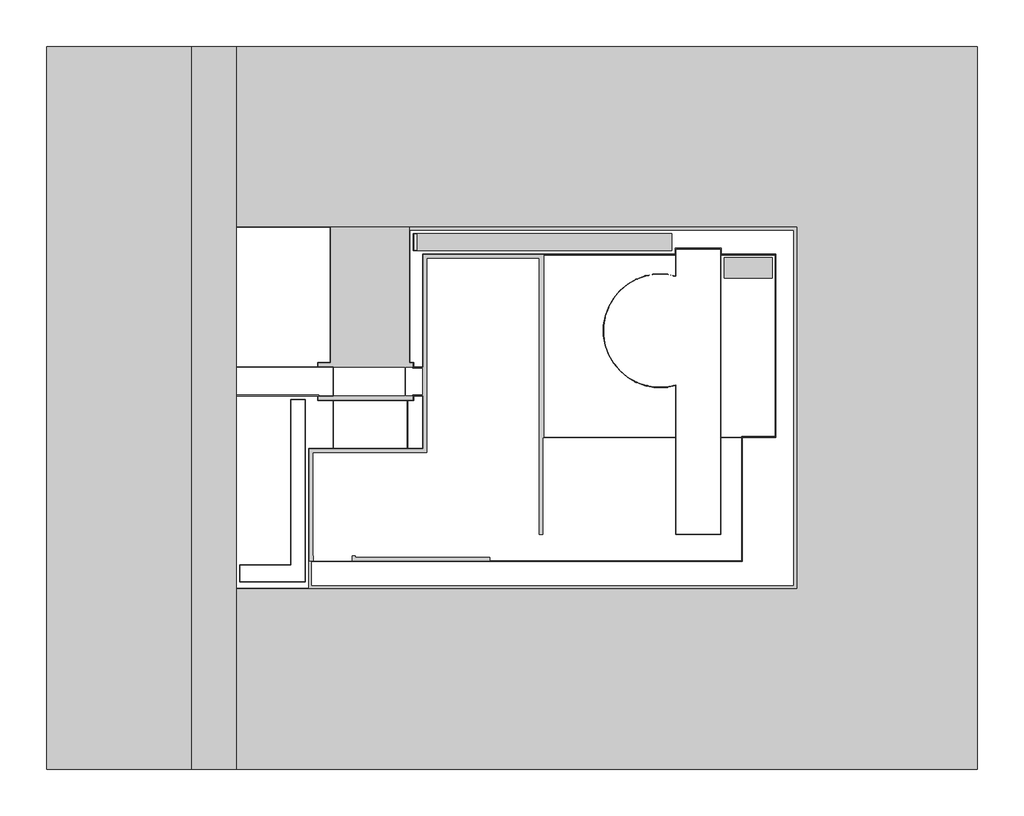
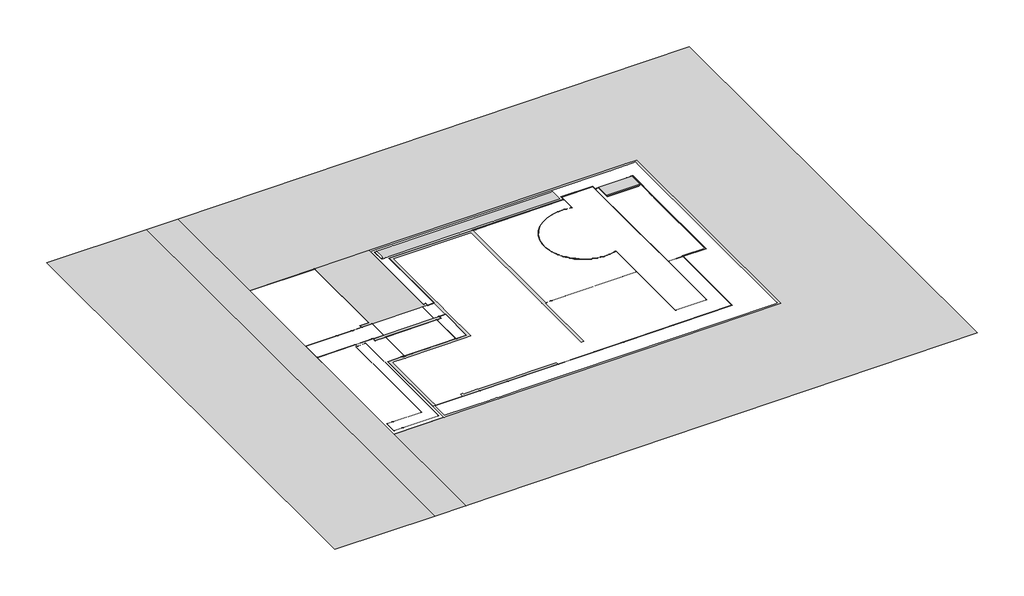
# One storey: 11 proxies.
"""IFC4 building model written with IfcOpenShell, lengths in millimetres."""

import ifcopenshell
import ifcopenshell.guid

model = None  # the IFC model being written
_history = None  # IfcOwnerHistory: only IFC2X3 demands one
_inside = {}  # id of a spatial element -> (the spatial element, [elements in it])
_under = {}  # id of a project, library or spatial element -> (it, [spatial elements below it])
_declared = {}  # id of a project -> (the project, [libraries it declares])
_typed = {}  # id of a type object -> (the type object, [elements of that type])
_made_of = {}  # id of a material, layer set ... -> (it, [elements and type objects made of it])


def new_model(schema):
    """Start an empty IFC model of exactly this schema.

    Asked for "IFC4X3", IfcOpenShell would pick the latest addendum, in which some entities
    have other attributes; the version numbers below select the first issue.
    IFC2X3 requires an IfcOwnerHistory on every rooted entity: one is made here for all.
    """
    global model, _history
    if schema == "IFC4X3":
        model = ifcopenshell.file(schema_version=(4, 3, 0, 0))
    else:
        model = ifcopenshell.file(schema=schema)
    _inside.clear()
    _under.clear()
    _declared.clear()
    _typed.clear()
    _made_of.clear()
    _history = None
    if model.schema == "IFC2X3":
        org = make("IfcOrganization", Name="unknown")
        user = make(
            "IfcPersonAndOrganization",
            ThePerson=make("IfcPerson", FamilyName="unknown"),
            TheOrganization=org,
        )
        app = make(
            "IfcApplication",
            ApplicationDeveloper=org,
            Version="unknown",
            ApplicationFullName="unknown",
            ApplicationIdentifier="unknown",
        )
        _history = make(
            "IfcOwnerHistory",
            OwningUser=user,
            OwningApplication=app,
            ChangeAction="ADDED",
            CreationDate=0,
        )
    return model


def make(cls, **values):
    """One entity of the class cls with the attributes given. An attribute that is None is left unset."""
    return model.create_entity(
        cls, **{name: value for name, value in values.items() if value is not None}
    )


def rooted(cls, **values):
    """An entity with a GlobalId (a new one), such as an element, a storey or a relation."""
    return make(cls, GlobalId=ifcopenshell.guid.new(), OwnerHistory=_history, **values)


def si_unit(unit_type, name, prefix=None):
    """IfcSIUnit, for example si_unit("LENGTHUNIT", "METRE", prefix="MILLI")."""
    return make("IfcSIUnit", UnitType=unit_type, Prefix=prefix, Name=name)


def assignment(units):
    """IfcUnitAssignment: the units of a project."""
    return None if units is None else make("IfcUnitAssignment", Units=units)


def point(xyz):
    """IfcCartesianPoint."""
    return None if xyz is None else make("IfcCartesianPoint", Coordinates=xyz)


def direction(xyz):
    """IfcDirection."""
    return None if xyz is None else make("IfcDirection", DirectionRatios=xyz)


def frame(location, z_axis=None, x_axis=None):
    """IfcAxis2Placement3D, a coordinate frame: its origin and axes. An axis left out is left unset."""
    return make(
        "IfcAxis2Placement3D",
        Location=point(location),
        Axis=direction(z_axis),
        RefDirection=direction(x_axis),
    )


def origin():
    """The frame at (0, 0, 0) with its axes left unset."""
    return frame((0.0, 0.0, 0.0))


def place(relative_to, where):
    """IfcLocalPlacement: puts the frame where relative to a parent placement (None: the world)."""
    return make(
        "IfcLocalPlacement", PlacementRelTo=relative_to, RelativePlacement=where
    )


def context(
    kind, dimensions, precision=None, world=None, true_north=None, identifier=None
):
    """IfcGeometricRepresentationContext, for example the 3D "Model" context."""
    return make(
        "IfcGeometricRepresentationContext",
        ContextIdentifier=identifier,
        ContextType=kind,
        CoordinateSpaceDimension=dimensions,
        Precision=precision,
        WorldCoordinateSystem=world,
        TrueNorth=true_north,
    )


def project(units=None, contexts=None):
    """IfcProject with its units and contexts."""
    return rooted(
        "IfcProject",
        Name="project",
        RepresentationContexts=contexts,
        UnitsInContext=assignment(units),
    )


def spatial(cls, under=None, at=None, **own):
    """A site, building, storey or space (cls), placed at a placement, below another one or the project."""
    s = rooted(cls, ObjectPlacement=at, **own)
    if under is not None:
        _under.setdefault(under.id(), (under, []))[1].append(s)
    return s


def polyline(points):
    """IfcPolyline through the points."""
    return make("IfcPolyline", Points=[point(p) for p in points])


def point_list(points):
    """IfcCartesianPointList2D or 3D."""
    cls = (
        "IfcCartesianPointList2D" if len(points[0]) == 2 else "IfcCartesianPointList3D"
    )
    return make(cls, CoordList=points)


def outline(outer, holes=None, kind="AREA"):
    """IfcArbitraryClosedProfileDef: a profile drawn as a closed curve; with holes, ...WithVoids."""
    if holes is None:
        return make("IfcArbitraryClosedProfileDef", ProfileType=kind, OuterCurve=outer)
    return make(
        "IfcArbitraryProfileDefWithVoids",
        ProfileType=kind,
        OuterCurve=outer,
        InnerCurves=holes,
    )


def extrude(swept, where, along, depth):
    """IfcExtrudedAreaSolid: the profile swept, set in the frame where, extruded along a direction by depth."""
    return make(
        "IfcExtrudedAreaSolid",
        SweptArea=swept,
        Position=where,
        ExtrudedDirection=direction(along),
        Depth=depth,
    )


def triangles(points, corners, closed=None, point_numbers=None):
    """IfcTriangulatedFaceSet: each triangle names its three corners, points numbered from 1."""
    return make(
        "IfcTriangulatedFaceSet",
        Coordinates=point_list(points),
        Closed=closed,
        CoordIndex=corners,
        PnIndex=point_numbers,
    )


def shape(context_of_items, identifier, shape_type, items):
    """IfcShapeRepresentation: the items that make up one representation, for example the "Body"."""
    return make(
        "IfcShapeRepresentation",
        ContextOfItems=context_of_items,
        RepresentationIdentifier=identifier,
        RepresentationType=shape_type,
        Items=items,
    )


def source(mapping_origin, context_of_items, identifier, shape_type, items):
    """IfcRepresentationMap: a shape defined once, which mapped items show again and again."""
    return make(
        "IfcRepresentationMap",
        MappingOrigin=mapping_origin,
        MappedRepresentation=shape(context_of_items, identifier, shape_type, items),
    )


def transform(
    local_origin,
    x_axis=None,
    y_axis=None,
    z_axis=None,
    scale=None,
    scale2=None,
    scale3=None,
    uniform=True,
):
    """IfcCartesianTransformationOperator3D, or its non-uniform kind. x_axis, y_axis, z_axis: its Axis1, 2, 3."""
    if uniform:
        return make(
            "IfcCartesianTransformationOperator3D",
            Axis1=direction(x_axis),
            Axis2=direction(y_axis),
            LocalOrigin=point(local_origin),
            Scale=scale,
            Axis3=direction(z_axis),
        )
    return make(
        "IfcCartesianTransformationOperator3DnonUniform",
        Axis1=direction(x_axis),
        Axis2=direction(y_axis),
        LocalOrigin=point(local_origin),
        Scale=scale,
        Axis3=direction(z_axis),
        Scale2=scale2,
        Scale3=scale3,
    )


def mapped(mapping_source, mapping_target):
    """IfcMappedItem: shows the shape of a source again, moved by a transform."""
    return make(
        "IfcMappedItem", MappingSource=mapping_source, MappingTarget=mapping_target
    )


def made_of(thing, what):
    """Note that an element or type object is made of a material, layer set ...; save() writes the relation."""
    if what is not None:
        _made_of.setdefault(what.id(), (what, []))[1].append(thing)
    return thing


def element(
    cls,
    number,
    at=None,
    inside=None,
    cuts=None,
    type_object=None,
    material=None,
    context=None,
    identifier="Body",
    shape_type=None,
    held_by="IfcProductDefinitionShape",
    body=None,
    shapes=None,
    **own,
):
    """One element of the class cls, such as IfcWall. Its Tag is "e" and its number.

    at: its placement. inside: the storey or other place that contains it. cuts: it is an
    opening in that element (IfcRelVoidsElement). A single representation is given by context,
    identifier, shape_type and body (its items); several are given by shapes. held_by: the class
    of the entity that holds the representations. save() writes the other relations.
    """
    e = rooted(cls, Tag="e%d" % number, ObjectPlacement=at, **own)
    if body is not None:
        shapes = [shape(context, identifier, shape_type, body)]
    if shapes is not None:
        e.Representation = make(held_by, Representations=shapes)
    if inside is not None:
        _inside.setdefault(inside.id(), (inside, []))[1].append(e)
    if cuts is not None:
        rooted(
            "IfcRelVoidsElement", RelatingBuildingElement=cuts, RelatedOpeningElement=e
        )
    if type_object is not None:
        _typed.setdefault(type_object.id(), (type_object, []))[1].append(e)
    return made_of(e, material)


def aggregate(whole, parts):
    """IfcRelAggregates: a whole, such as a stair, and the parts it consists of."""
    return rooted("IfcRelAggregates", RelatingObject=whole, RelatedObjects=parts)


def save(model, path):
    """Write the relations noted so far, then the file.

    IfcRelAggregates (storeys below a building ...), IfcRelContainedInSpatialStructure (elements
    in a storey), IfcRelDefinesByType, IfcRelAssociatesMaterial and IfcRelDeclares: one each for
    every whole, place, type object, material and project.
    """
    for whole, parts in _under.values():
        aggregate(whole, parts)
    for where, things in _inside.values():
        rooted(
            "IfcRelContainedInSpatialStructure",
            RelatedElements=things,
            RelatingStructure=where,
        )
    for kind, things in _typed.values():
        rooted("IfcRelDefinesByType", RelatedObjects=things, RelatingType=kind)
    for what, things in _made_of.values():
        rooted("IfcRelAssociatesMaterial", RelatedObjects=things, RelatingMaterial=what)
    for by, libraries in _declared.values():
        rooted("IfcRelDeclares", RelatingContext=by, RelatedDefinitions=libraries)
    model.write(path)


def specialty_equipment_67e2e29c(model_context):
    return source(origin(), model_context, "Body", "SweptSolid", [
        extrude(outline(polyline([(12687.718693, 5627.4300153), (12687.718693, 4481.4300153), (10041.718693, 4481.4300153), (10041.718693, 5627.4300153), (12687.718693, 5627.4300153)])), frame((0.0, 0.0, 280.0), z_axis=(0.0, 0.0, 1.0), x_axis=(1.0, 0.0, 0.0)), (0.0, 0.0, 1.0), 88.4706632),
        extrude(outline(polyline([(12614.718693, 5554.4300153), (12614.718693, 4554.4300153), (10114.718693, 4554.4300153), (10114.718693, 5554.4300153), (12614.718693, 5554.4300153)])), frame((0.0, 0.0, 200.0), z_axis=(0.0, 0.0, 1.0), x_axis=(1.0, 0.0, 0.0)), (0.0, 0.0, 1.0), 80.0),
    ])


model = new_model("IFC4")

# Units and contexts
model_context = context("Model", 3, world=origin())
ifc_project = project(units=[si_unit("LENGTHUNIT", "METRE", prefix="MILLI")], contexts=[model_context])

# Site, building, storey
site = spatial("IfcSite", under=ifc_project)
building = spatial("IfcBuilding", under=site)
storey = spatial("IfcBuildingStorey", under=building, Name="NÍVEL DA RUA", Elevation=0.0)

# Proxies
placement = place(None, origin())
element("IfcBuildingElementProxy", 1, Name="Building Element Proxy", at=placement, inside=storey, context=model_context, shape_type="Tessellation", body=[
    triangles([(24039.718689, -22695.5705017, 300.0000023), (24039.718689, 17304.4298035, 300.0000023), (-16960.2810425, 17304.4298035, 17.2413792), (-16960.2810425, 16538.146344, 17.2413792), (-16960.2810425, 7304.4297272, 17.2413792), (13164.7185333, 7304.4297272, 225.0000017), (14039.7186127, 7304.4297272, 231.0344808), (14039.7186127, -12695.5704254, 231.0344808), (-8585.2811966, -12695.5704254, 75.0000006), (-16960.2810425, -12695.5704254, 17.2413792), (-16960.2810425, -20396.7201233, 17.2413792), (-16960.2810425, -22695.5705017, 17.2413792)], [[11, 9, 10], [9, 11, 12], [6, 3, 4], [6, 4, 5], [12, 8, 9], [8, 12, 1], [8, 1, 7], [6, 7, 2], [2, 7, 1], [2, 3, 6]], closed=False),
])
element("IfcBuildingElementProxy", 2, Name="Building Element Proxy", at=placement, inside=storey, context=model_context, shape_type="Tessellation", body=[
    triangles([(-27460.2819946, 17304.4298035, 0.0), (-27460.2819946, -22695.5705017, 0.0), (-19460.2807709, -22695.5705017, 0.0), (-19460.2807709, -15076.5227692, 13.1362894), (-19460.2807709, 161.5728776, 13.1362894), (-19460.2807709, 9685.3826523, 13.1362894), (-19460.2807709, 17304.4298035, 0.0)], [[1, 2, 5], [5, 2, 4], [1, 5, 6], [3, 4, 2], [6, 7, 1]], closed=False),
])
element("IfcBuildingElementProxy", 3, Name="Building Element Proxy", at=placement, inside=storey, context=model_context, shape_type="Tessellation", body=[
    triangles([(-19460.2807709, -22695.5705017, 0.0), (-16960.2810425, -22695.5705017, 17.2413792), (-16960.2810425, -20396.7201233, 17.2413792), (-16960.2810425, -12695.5704254, 17.2413792), (-16960.2810425, 7304.4297272, 17.2413792), (-16960.2810425, 16538.146344, 17.2413792), (-16960.2810425, 17304.4298035, 17.2413792), (-19460.2807709, 17304.4298035, 0.0), (-19460.2807709, 9685.3826523, 13.1362894), (-19460.2807709, 161.5728776, 13.1362894), (-19460.2807709, -15076.5227692, 13.1362894)], [[10, 11, 4], [6, 8, 9], [5, 9, 10], [11, 1, 3], [11, 3, 4], [3, 1, 2], [6, 7, 8], [6, 9, 5], [4, 5, 10]], closed=False),
])
element("IfcBuildingElementProxy", 4, Name="Building Element Proxy", at=placement, inside=storey, context=model_context, shape_type="Tessellation", body=[
    triangles([(14039.7186127, 7304.4297272, 231.0344808), (13164.7185333, 7304.4297272, 225.0000017), (-7360.2815506, 7304.4297272, 83.4482767), (-7360.2815506, 7054.4298706, 83.4482767), (-7360.2815506, -195.5699849, 83.4482767), (-7160.2815491, -195.5699849, 84.8275893), (-7160.2815491, -445.5699686, 84.8275893), (-6660.2812546, -445.5699686, 88.2758617), (-6660.2812546, 5804.4300064, 88.2758617), (39.7186921, 5804.4300064, 134.4827615), (7339.7188522, 5804.4300064, 184.827581), (7339.7188522, 6104.4302994, 184.827581), (9839.719162, 6104.4302994, 202.0689704), (9839.719162, 5804.4300064, 202.0689704), (12414.7189636, 5804.4300064, 219.8275885), (12736.6074554, 5804.4300064, 222.0475111), (12889.7190399, 5804.4300064, 223.1034423), (12889.7190399, 5796.7827988, 223.1034423), (12889.7190399, 2838.5967934, 223.1034423), (12889.7190399, -4345.5699257, 223.1034423), (11039.7191711, -4345.5699257, 210.3448279), (11039.7191711, -11195.5701233, 210.3448279), (-6954.0313477, -11195.5701233, 86.2500043), (-9213.4062286, -11195.5701233, 70.668102), (-12960.281012, -11195.5701233, 44.8275872), (-12960.281012, -4945.5702209, 44.8275872), (-11830.5941528, -4945.5702209, 52.618536), (-11610.2808563, -4945.5702209, 54.1379291), (-11610.2808563, -4820.5615723, 54.1379291), (-11610.2808563, -2295.5700554, 54.1379291), (-12460.2812988, -2295.5700554, 48.2758642), (-12460.2812988, -2045.5700535, 48.2758642), (-13907.2197235, -2045.5700535, 38.296972), (-16960.2810425, -2045.5700535, 17.2413792), (-16960.2810425, -12695.5704254, 17.2413792), (-8585.2811966, -12695.5704254, 75.0000006), (14039.7186127, -12695.5704254, 231.0344808), (-12461.2812378, -2046.5183968, 48.2689651), (-12461.2812378, -2051.3699902, 48.2689651), (-12461.2812378, -2296.5699944, 48.2689651), (-12460.4696594, -2296.5699944, 48.2745606), (-11611.2807953, -2296.5699944, 54.1310346), (-11611.2807953, -4821.1289795, 54.1310346), (-11611.2807953, -4944.5697006, 54.1310346), (-11828.8314697, -4944.5697006, 52.6306901), (-11830.8313477, -4944.5697006, 52.6168964), (-12960.0926514, -4944.5697006, 44.8288862), (-12961.2809509, -4944.5697006, 44.8206881), (-12961.2809509, -4947.507312, 44.8206881), (-12961.2809509, -11195.944519, 44.8206881), (-12961.2809509, -12694.5704865, 44.8206881), (-16957.6149261, -12694.5704865, 17.2597704), (-16959.2811035, -12694.5704865, 17.2482761), (-16959.2811035, -12693.6321716, 17.2482761), (-16959.2811035, -2046.5183968, 17.2482761), (-13906.9104401, -2046.5183968, 38.2991112), (13889.7184662, 7154.430162, 230.0000054), (13889.7184662, 6721.9298172, 230.0000054), (13889.7184662, -12278.0703278, 230.0000054), (13889.7184662, -12545.5702789, 230.0000054), (13739.7183197, -12545.5702789, 228.9655118), (-6622.781218, -12545.5702789, 88.5344851), (-8422.1562698, -12545.5702789, 76.125), (-8648.0936417, -12545.5702789, 74.5668103), (-9022.7812363, -12545.5702789, 71.9827565), (-12809.2809265, -12545.5702789, 45.8689662), (-12809.2809265, -11247.3413818, 45.8689662), (-12809.2809265, -11196.5700623, 45.8689662), (-9212.9876495, -11196.5700623, 70.6709906), (-6955.119072, -11196.5700623, 86.2425011), (9.7186928, -11196.5700623, 134.275861), (2289.7186684, -11196.5700623, 150.0000011), (6259.7184952, -11196.5700623, 177.3793074), (11026.6350861, -11196.5700623, 210.25459), (11040.7191101, -11196.5700623, 210.3517316), (11040.7191101, -4348.353186, 210.3517316), (11040.7191101, -4346.5698647, 210.3517316), (12890.7189789, -4346.5698647, 223.110346), (12890.7189789, 2842.4799866, 223.110346), (12890.7189789, 5802.2650223, 223.110346), (12890.7189789, 5805.4299454, 223.110346), (12736.8923218, 5805.4299454, 222.0494732), (12415.2189331, 5805.4299454, 219.8310403), (9870.7184326, 5805.4299454, 202.2827655), (9870.7184326, 6135.4301514, 202.2827655), (7308.7184189, 6135.4301514, 184.6137859), (7308.7184189, 5805.4299454, 184.6137859), (48.468694, 5805.4299454, 134.5431049), (34.7853586, 5805.4299454, 134.4487338), (-6661.2811935, 5805.4299454, 88.2689672), (-6661.2811935, 5795.8584366, 88.2689672), (-6661.2811935, 5792.4301575, 88.2689672), (-6661.2811935, -444.5699933, 88.2689672), (-6662.2811325, -444.5699933, 88.2620726), (-7159.2810287, -444.5699933, 84.8344839), (-7159.2810287, -196.0699907, 84.8344839), (-7159.2810287, -194.5699914, 84.8344839), (-7160.1978333, -194.5699914, 84.8281616), (-7359.2810303, -194.5699914, 83.4551713), (-7359.2810303, -186.9985604, 83.4551713), (-7359.2810303, 7154.430162, 83.4551713), (-7290.2811722, 7154.430162, 83.9310325), (-6620.2813705, 7154.430162, 88.5517261), (11852.2184143, 7154.430162, 215.9482831), (13089.7184601, 7154.430162, 224.4827549), (13121.907193, 7154.430162, 224.7047436), (13137.3585754, 7154.430162, 224.8113141), (-12460.2812988, -445.5699686, 48.2758642), (-12460.2812988, -195.5699849, 48.2758642), (-11760.2810028, -195.5699849, 53.1034492), (-11760.2810028, 7054.4298706, 53.1034492), (-11760.2810028, 7304.4297272, 53.1034492), (-16960.2810425, 7304.4297272, 17.2413792), (-16960.2810425, -445.5699686, 17.2413792), (-14429.6692291, -445.5699686, 34.6938784), (-13230.3342957, -445.5699686, 42.9651464), (-11761.2809418, 7303.4297882, 53.0965501), (-11761.2809418, 7293.7158463, 53.0965501), (-11761.2809418, -194.5699914, 53.0965501), (-12460.1882813, -194.5699914, 48.2765046), (-12461.2812378, -194.5699914, 48.2689651), (-12461.2812378, -439.5699715, 48.2689651), (-12463.7648071, -439.5699715, 48.2518331), (-13233.2224915, -439.5699715, 42.9452348), (-14431.6284119, -439.5699715, 34.6803663), (-16959.2811035, -439.5699715, 17.2482761), (-16959.2811035, 7301.3677048, 17.2482761), (-16959.2811035, 7302.351947, 17.2482761), (-16959.2811035, 7303.4297882, 17.2482761), (-6660.2812546, -4945.5702209, 88.2758617), (-6660.2812546, -2045.5700535, 88.2758617), (-7160.2815491, -2045.5700535, 84.8275893), (-7160.2815491, -2295.5700554, 84.8275893), (-7510.2811157, -2295.5700554, 82.4137922), (-7510.2811157, -2494.1649101, 82.4137922), (-7510.2811157, -4945.5702209, 82.4137922), (-6661.2811935, -2046.5699924, 88.2689672), (-6661.2811935, -4940.2699631, 88.2689672), (-6661.2811935, -4944.5697006, 88.2689672), (-7484.2815399, -4944.5697006, 82.5931054), (-7484.2815399, -2479.4120316, 82.5931054), (-7484.2815399, -2296.5699944, 82.5931054), (-7162.0436508, -2296.5699944, 84.8154352), (-7160.0926071, -2296.5699944, 84.8288883), (-7159.2810287, -2296.5699944, 84.8344839), (-7159.2810287, -2295.0699406, 84.8344839), (-7159.2810287, -2046.5699924, 84.8344839), (-6662.2811325, -2046.5699924, 88.2620726), (-7159.2810287, 6005.4299469, 84.8344839), (-6960.2815475, 6005.4299469, 86.2068928), (-6960.2815475, 6447.2872787, 86.2068928), (-6960.2815475, 6953.4302216, 86.2068928), (-7159.2810287, 6953.4302216, 84.8344839), (-7159.2810287, 6873.7159012, 84.8344839), (7140.7187897, 6955.4300995, 183.455172), (-5638.5476898, 6955.4300995, 95.3222975), (-7161.281488, 6955.4300995, 84.8206856), (-7161.281488, 6878.0016861, 84.8206856), (-7161.281488, 6003.430069, 84.8206856), (-6753.1482605, 6003.430069, 87.635403), (-942.0146662, 6003.430069, 127.712181), (1780.9687626, 6003.430069, 146.4913763), (7140.7187897, 6003.430069, 183.455172), (7140.7187897, 6615.9729126, 183.455172), (-6960.2815475, 6954.4301605, 86.2068928), (-5633.6148514, 6954.4301605, 95.3563253), (7139.7188507, 6954.4301605, 183.4482684), (7139.7188507, 6615.8583847, 183.4482684), (7139.7188507, 6004.4300079, 183.4482684), (1789.7186646, 6004.4300079, 146.5517196), (-946.9479406, 6004.4300079, 127.6781623), (-6753.6145111, 6004.4300079, 87.6321874), (-6960.2815475, 6004.4300079, 86.2068928)], [[35, 53, 54], [53, 35, 52], [51, 52, 35], [35, 36, 51], [34, 35, 54], [66, 67, 50], [67, 25, 50], [25, 67, 68], [68, 24, 25], [66, 50, 51], [51, 65, 66], [49, 50, 25], [49, 26, 48], [49, 25, 26], [47, 48, 26], [26, 46, 47], [31, 41, 42], [39, 40, 31], [31, 40, 41], [30, 31, 42], [39, 32, 38], [46, 26, 27], [45, 46, 27], [68, 69, 24], [45, 28, 44], [45, 27, 28], [29, 44, 28], [65, 36, 64], [36, 65, 51], [64, 36, 63], [70, 24, 69], [36, 62, 63], [140, 135, 136], [43, 44, 29], [29, 30, 42], [31, 32, 39], [43, 29, 42], [140, 141, 135], [141, 142, 134], [142, 143, 133], [133, 143, 144], [142, 133, 134], [133, 147, 132], [141, 134, 135], [33, 55, 56], [55, 33, 34], [125, 114, 115], [55, 34, 54], [33, 38, 32], [123, 116, 108], [122, 108, 109], [115, 116, 124], [33, 56, 38], [108, 122, 123], [126, 127, 113], [113, 128, 129], [128, 113, 127], [113, 129, 112], [126, 113, 114], [115, 124, 125], [125, 126, 114], [123, 124, 116], [121, 109, 120], [121, 122, 109], [109, 119, 120], [5, 100, 4], [100, 5, 99], [99, 6, 98], [5, 6, 99], [119, 109, 110], [98, 6, 97], [154, 159, 149], [95, 6, 7], [118, 111, 112], [118, 112, 117], [117, 112, 129], [157, 158, 153], [154, 158, 159], [153, 158, 154], [157, 165, 156], [100, 101, 4], [101, 102, 3], [101, 3, 4], [102, 103, 3], [119, 110, 111], [153, 165, 157], [119, 111, 118], [133, 144, 145], [146, 147, 133], [130, 140, 136], [24, 70, 23], [139, 140, 130], [138, 139, 130], [131, 137, 138], [23, 71, 72], [148, 137, 131], [7, 94, 95], [7, 8, 94], [97, 6, 96], [95, 96, 6], [147, 148, 132], [94, 8, 93], [93, 8, 92], [91, 92, 9], [8, 9, 92], [91, 9, 90], [148, 131, 132], [70, 71, 23], [73, 22, 72], [22, 76, 21], [74, 75, 22], [61, 37, 60], [60, 37, 59], [22, 75, 76], [58, 59, 37], [37, 61, 62], [73, 74, 22], [131, 138, 130], [87, 10, 11], [89, 9, 10], [21, 77, 20], [21, 76, 77], [20, 78, 19], [19, 78, 79], [18, 79, 80], [18, 19, 79], [78, 20, 77], [17, 18, 80], [58, 37, 1], [23, 72, 22], [62, 36, 37], [90, 9, 89], [160, 173, 159], [172, 150, 173], [172, 173, 160], [152, 166, 165], [161, 171, 160], [149, 159, 173], [156, 165, 166], [89, 10, 88], [162, 163, 170], [163, 169, 170], [170, 171, 162], [87, 88, 10], [162, 171, 161], [172, 171, 166], [170, 166, 171], [149, 173, 150], [160, 171, 172], [165, 153, 152], [166, 151, 172], [151, 150, 172], [168, 167, 170], [169, 163, 164], [170, 167, 166], [166, 155, 156], [167, 155, 166], [167, 168, 164], [152, 151, 166], [168, 170, 169], [11, 12, 87], [84, 13, 14], [12, 13, 86], [13, 85, 86], [13, 84, 85], [168, 169, 164], [17, 82, 16], [15, 16, 83], [16, 82, 83], [82, 17, 81], [80, 81, 17], [84, 15, 83], [104, 105, 2], [2, 3, 104], [164, 155, 167], [106, 107, 2], [2, 57, 1], [57, 2, 107], [1, 57, 58], [106, 2, 105], [103, 104, 3], [87, 12, 86], [15, 84, 14], [133, 145, 146]], closed=False),
])
element("IfcBuildingElementProxy", 5, Name="Building Element Proxy", at=placement, inside=storey, context=model_context, shape_type="Tessellation", body=[
    triangles([(-7510.2811157, -2295.5700554, 82.4137922), (-11610.2808563, -2295.5700554, 54.1379291), (-11610.2808563, -4820.5615723, 54.1379291), (-11610.2808563, -4945.5702209, 54.1379291), (-7510.2811157, -4945.5702209, 82.4137922), (-7510.2811157, -2494.1649101, 82.4137922), (-7511.2810547, -2296.5699944, 82.4068977), (-7511.2810547, -2494.1163666, 82.4068977), (-7511.2810547, -4944.5697006, 82.4068977), (-7543.0791138, -4944.5697006, 82.1875978), (-11609.2809174, -4944.5697006, 54.1448282), (-11609.2809174, -4820.5920937, 54.1448282), (-11609.2809174, -2296.5699944, 54.1448282), (-11589.6367676, -2296.5699944, 54.2803123)], [[3, 4, 11], [11, 4, 10], [3, 11, 12], [2, 3, 13], [13, 14, 2], [13, 3, 12], [2, 14, 1], [10, 5, 9], [5, 10, 4], [9, 5, 6], [9, 6, 8], [7, 8, 6], [6, 1, 7], [7, 1, 14]], closed=False),
])
element("IfcBuildingElementProxy", 6, Name="Building Element Proxy", at=placement, inside=storey, context=model_context, shape_type="Tessellation", body=[
    triangles([(7339.7188522, -4345.5699257, 184.827581), (7339.7188522, -9695.5698212, 184.827581), (9839.719162, -9695.5698212, 202.0689704), (9839.719162, -4345.5699257, 202.0689704), (9839.719162, 654.4300398, 202.0689704), (9839.719162, 6104.4302994, 202.0689704), (7339.7188522, 6104.4302994, 184.827581), (7339.7188522, 4607.5800957, 184.827581), (6796.6921143, 4709.4366692, 181.0825697), (6244.2217667, 4714.8491295, 177.272428), (5699.3044464, 4623.6503357, 173.5143907), (5178.7025024, 4438.6465118, 169.9240212), (4698.432399, 4165.5288803, 166.6118142), (4273.2688156, 3812.6995445, 163.6796531), (3916.2914772, 3391.0127838, 161.2177394), (3638.4822716, 2913.4410622, 159.3018135), (3448.3874794, 2394.6766514, 157.9908106), (3351.8552902, 1850.6783157, 157.3250809), (3351.8552902, 1298.1816616, 157.3250809), (3375.1727623, 1166.7781271, 157.4858814), (3448.3874794, 754.1833986, 157.9908106), (3638.4822716, 235.4189333, 159.3018135), (3916.2914772, -242.152643, 161.2177394), (4273.2688156, -663.8394218, 163.6796531), (4698.432399, -1016.6688303, 166.6118142), (5116.5376923, -1254.4350586, 169.4953046), (5178.7025024, -1289.7865345, 169.9240212), (5699.3044464, -1474.7903584, 173.5143907), (6244.2217667, -1565.9890068, 177.272428), (6796.6921143, -1560.5766918, 181.0825697), (7339.7188522, -1458.7201183, 184.827581), (9838.719223, 6103.4297791, 202.0620668), (9838.719223, 656.0112659, 202.0620668), (9838.719223, 653.5847425, 202.0620668), (9838.719223, -4344.415345, 202.0620668), (9838.719223, -4345.5699257, 202.0620668), (9838.719223, -4347.7099113, 202.0620668), (9838.719223, -9694.5698822, 202.0620668), (7340.7187912, -9694.5698822, 184.8344846), (7340.7187912, -9693.4298355, 184.8344846), (7340.7187912, -4345.5699257, 184.8344846), (7340.7187912, -1459.8748444, 184.8344846), (7340.7187912, -1457.8749664, 184.8344846), (7340.7187912, -1447.0134201, 184.8344846), (7339.7188522, -1447.2022167, 184.827581), (7298.6940308, -1454.9504356, 184.5446586), (6799.331488, -1549.2634289, 181.1007736), (6738.2637039, -1549.930394, 180.6796147), (6248.4058136, -1555.2806488, 177.3012962), (6140.4943771, -1537.3313084, 176.5570647), (5704.9145691, -1464.8797714, 173.5530693), (5198.0809708, -1285.2682056, 170.0576795), (5185.6009186, -1280.8455105, 169.9716019), (5184.0382233, -1279.9583553, 169.9608285), (5160.4478027, -1266.5664402, 169.7981386), (5149.7327591, -1260.4835266, 169.7242332), (5143.4308182, -1256.906274, 169.6807766), (5120.5310532, -1243.9063408, 169.5228466), (5100.9851532, -1232.8106518, 169.3880437), (5070.1288971, -1215.2939157, 169.1752479), (5020.0999741, -1186.8933964, 168.8302108), (4706.4641762, -1008.8477234, 166.6672069), (4382.4897652, -740.3338079, 164.4328956), (4282.2644875, -657.2659132, 163.7416951), (3966.0765198, -284.1410139, 161.5610869), (3926.0708221, -236.9313229, 161.2851771), (3891.4450287, -177.4590991, 161.0463836), (3648.8563477, 239.2065837, 159.3733571), (3598.8945717, 375.4450702, 159.0287923), (3459.1615311, 756.4792614, 158.0651157), (3405.0970985, 1060.9314629, 157.6922642), (3395.8714989, 1112.8837423, 157.6286416), (3389.9497673, 1146.2321428, 157.5878011), (3384.815197, 1175.1465843, 157.5523926), (3384.5727699, 1176.5109632, 157.5507212), (3384.2972054, 1178.0621767, 157.5488136), (3383.976004, 1179.8718773, 157.5465972), (3383.5896904, 1182.0475439, 157.5439447), (3383.1077431, 1184.7605324, 157.5406201), (3382.4787117, 1188.3028307, 157.5362781), (3381.6055092, 1193.2199724, 157.5302464), (3380.2823341, 1200.6721338, 157.5211264), (3377.9699753, 1213.692778, 157.5051753), (3372.528447, 1244.3365471, 157.4676594), (3362.8302017, 1298.9508007, 157.4007667), (3362.8302017, 1528.7872078, 157.4007667), (3362.8302017, 1849.9091766, 157.4007667), (3442.7352081, 2299.8790947, 157.9518414), (3459.1615311, 2392.3808613, 158.0651157), (3630.2714355, 2858.9754913, 159.2451854), (3648.8563477, 2909.6535027, 159.3733571), (3907.090004, 3353.1906738, 161.1542803), (3926.0708221, 3385.7913002, 161.2851771), (4263.5359795, 3784.025132, 163.6125242), (4282.2644875, 3806.1258179, 163.7416951), (4688.3600487, 4142.702948, 166.5423599), (4706.4641762, 4157.7078461, 166.6672069), (5168.3874344, 4419.9337006, 169.8528955), (5185.6009186, 4429.7054878, 169.9716019), (5688.8021805, 4608.0297775, 173.4419569), (5704.9145691, 4613.7398941, 173.5530693), (6233.5671844, 4701.6726082, 177.1989587), (6248.4058136, 4704.1407715, 177.3012962), (6785.9073074, 4698.2701996, 181.008192), (6799.331488, 4698.1234062, 181.1007736), (7328.8195175, 4598.1207893, 184.752422), (7335.6423569, 4596.8322052, 184.7994759), (7339.7188522, 4596.0621941, 184.827581), (7340.7187912, 4595.8732521, 184.8344846), (7340.7187912, 4605.9987968, 184.8344846), (7340.7187912, 4608.1788963, 184.8344846), (7340.7187912, 6103.4297791, 184.8344846)], [[21, 69, 70], [69, 21, 22], [21, 70, 71], [23, 67, 22], [22, 68, 69], [68, 22, 67], [20, 75, 76], [75, 20, 74], [20, 76, 77], [71, 72, 20], [73, 74, 20], [72, 73, 20], [20, 21, 71], [67, 23, 66], [60, 61, 26], [59, 60, 26], [56, 57, 26], [26, 58, 59], [58, 26, 57], [56, 26, 27], [61, 25, 26], [23, 65, 66], [65, 23, 24], [65, 24, 64], [25, 62, 63], [62, 25, 61], [64, 24, 63], [63, 24, 25], [84, 20, 83], [83, 20, 82], [79, 20, 78], [81, 20, 80], [80, 20, 79], [20, 81, 82], [87, 18, 86], [86, 18, 19], [18, 87, 88], [84, 85, 19], [85, 86, 19], [20, 84, 19], [18, 88, 17], [78, 20, 77], [17, 89, 90], [89, 17, 88], [17, 90, 16], [16, 91, 92], [91, 16, 90], [16, 92, 15], [15, 92, 93], [15, 94, 14], [15, 93, 94], [14, 94, 95], [96, 13, 14], [13, 97, 98], [97, 13, 96], [96, 14, 95], [28, 29, 50], [50, 29, 49], [51, 28, 50], [29, 48, 49], [48, 29, 30], [47, 48, 30], [30, 46, 47], [27, 52, 53], [27, 28, 52], [27, 53, 54], [46, 30, 31], [45, 46, 31], [31, 43, 45], [28, 51, 52], [2, 39, 40], [39, 2, 38], [1, 2, 40], [38, 3, 37], [3, 38, 2], [37, 4, 36], [4, 37, 3], [42, 43, 31], [42, 1, 41], [43, 44, 45], [41, 1, 40], [36, 4, 35], [1, 42, 31], [35, 4, 5], [55, 56, 27], [98, 99, 12], [98, 12, 13], [100, 11, 12], [100, 12, 99], [55, 27, 54], [11, 100, 101], [11, 102, 10], [11, 101, 102], [10, 102, 103], [104, 105, 9], [104, 10, 103], [10, 104, 9], [105, 106, 9], [8, 106, 107], [108, 110, 107], [34, 5, 33], [5, 34, 35], [5, 6, 33], [110, 108, 109], [110, 8, 107], [111, 8, 110], [112, 8, 111], [8, 112, 7], [6, 7, 32], [6, 32, 33], [32, 7, 112], [9, 106, 8]], closed=False),
])
element("IfcBuildingElementProxy", 7, Name="Building Element Proxy", at=placement, inside=storey, context=model_context, shape_type="Tessellation", body=[
    triangles([(39.7186921, 5804.4300064, 134.4827615), (39.7186921, -4345.5699257, 134.4827615), (495.343711, -4345.5699257, 137.6250025), (7339.7188522, -4345.5699257, 184.827581), (7339.7188522, -1458.7201183, 184.827581), (6796.6921143, -1560.5766918, 181.0825697), (6244.2217667, -1565.9890068, 177.272428), (5699.3044464, -1474.7903584, 173.5143907), (5178.7025024, -1289.7865345, 169.9240212), (5116.5376923, -1254.4350586, 169.4953046), (4698.432399, -1016.6688303, 166.6118142), (4273.2688156, -663.8394218, 163.6796531), (3916.2914772, -242.152643, 161.2177394), (3638.4822716, 235.4189333, 159.3018135), (3448.3874794, 754.1833986, 157.9908106), (3375.1727623, 1166.7781271, 157.4858814), (3351.8552902, 1298.1816616, 157.3250809), (3351.8552902, 1850.6783157, 157.3250809), (3448.3874794, 2394.6766514, 157.9908106), (3638.4822716, 2913.4410622, 159.3018135), (3916.2914772, 3391.0127838, 161.2177394), (4273.2688156, 3812.6995445, 163.6796531), (4698.432399, 4165.5288803, 166.6118142), (5178.7025024, 4438.6465118, 169.9240212), (5699.3044464, 4623.6503357, 173.5143907), (6244.2217667, 4714.8491295, 177.272428), (6796.6921143, 4709.4366692, 181.0825697), (7339.7188522, 4607.5800957, 184.827581), (7339.7188522, 5804.4300064, 184.827581), (7338.7189133, -1460.0386425, 184.8206955), (7338.7189133, -4340.4414597, 184.8206955), (7338.7189133, -4343.0325806, 184.8206955), (7338.7189133, -4344.5699867, 184.8206955), (496.8763209, -4344.5699867, 137.6355669), (496.0298246, -4344.5699867, 137.6297351), (40.7045512, -4344.5699867, 134.4895562), (40.7045512, 5754.4301514, 134.4895562), (76.4691787, 5754.4301514, 134.7362072), (81.6046937, 5754.4301514, 134.7716247), (89.7027914, 5754.4301514, 134.8274807), (101.9597376, 5754.4301514, 134.9120049), (120.031636, 5754.4301514, 135.0366431), (145.9968752, 5754.4301514, 135.215711), (181.8478755, 5754.4301514, 135.4629615), (227.8518807, 5754.4301514, 135.7802296), (7260.6062393, 5754.4301514, 184.2819747), (7270.2556503, 5754.4301514, 184.3485223), (7289.4475021, 5754.4301514, 184.4808907), (7314.9226913, 5754.4301514, 184.6565885), (7338.7189133, 5754.4301514, 184.8206955), (7338.7189133, 4608.8986198, 184.8206955), (6797.103717, 4710.266851, 181.085422), (6795.6020645, 4710.5479385, 181.0750666), (6245.1211304, 4715.743261, 177.2786413), (6243.0799759, 4715.7624458, 177.2645615), (5700.982251, 4624.8584015, 173.5259634), (5698.1417267, 4624.3819771, 173.5063607), (5182.2540298, 4440.8911423, 169.9485291), (5177.5438522, 4439.2159538, 169.9160457), (4697.2955498, 4165.9585052, 166.603984), (4272.1636505, 3813.0123161, 163.6720409), (3915.2211937, 3391.2302124, 161.2103634), (3637.4436722, 2913.5820419, 159.2946555), (3447.3730064, 2394.755135, 157.9838161), (3351.0251083, 1851.6695343, 157.3193582), (3350.8536072, 1850.7034595, 157.3181773), (3350.8536072, 1299.5445145, 157.3181773), (3350.8536072, 1298.1565178, 157.3181773), (3351.082663, 1296.8651722, 157.3197578), (3374.3905426, 1165.4854734, 157.4805038), (3447.3730064, 754.104915, 157.9838161), (3447.7136833, 753.1751026, 157.9861779), (3637.4436722, 235.2780444, 159.2946555), (3637.8384155, 234.5993068, 159.2973806), (3915.2211937, -242.3702169, 161.2103634), (4272.1636505, -664.1523388, 163.6720409), (4697.2955498, -1017.0985279, 166.603984), (5115.5615891, -1255.0883617, 169.4885645), (5177.5438522, -1290.3559765, 169.9160457), (5179.6297714, -1291.0977917, 169.9304162), (5698.1417267, -1475.5218544, 173.5063607), (5699.8898758, -1475.8150051, 173.5184239), (6243.0799759, -1566.9026138, 177.2645615), (6244.5763962, -1566.8883705, 177.2748806), (6795.6020645, -1561.6879612, 181.0750666), (6796.8630341, -1561.4520744, 181.0837506), (9839.719162, -4345.5699257, 202.0689704), (11039.7191711, -4345.5699257, 210.3448279), (12889.7190399, -4345.5699257, 223.1034423), (12889.7190399, 2838.5967934, 223.1034423), (12889.7190399, 5796.7827988, 223.1034423), (12889.7190399, 5804.4300064, 223.1034423), (12736.6074554, 5804.4300064, 222.0475111), (12414.7189636, 5804.4300064, 219.8275885), (9839.719162, 5804.4300064, 202.0689704), (9839.719162, 654.4300398, 202.0689704), (12839.7186035, 5754.4301514, 222.7586233), (12839.7186035, 3807.1167458, 222.7586233), (12839.7186035, 3150.7896561, 222.7586233), (12839.7186035, 2887.2167908, 222.7586233), (12839.7186035, 2802.7905487, 222.7586233), (12839.7186035, -4263.6028358, 222.7586233), (12839.7186035, -4295.5700706, 222.7586233), (11027.7187408, -4295.5700706, 210.262075), (10989.7187347, -4295.5700706, 210.0000089), (10989.7187347, -4344.5699867, 210.0000089), (9840.719101, -4344.5699867, 202.0758559), (9840.719101, 650.263361, 202.0758559), (9840.719101, 652.7906776, 202.0758559), (9840.719101, 655.1461298, 202.0758559), (9840.719101, 5754.4301514, 202.0758559), (9891.1381165, 5754.4301514, 202.4235818), (12422.7266144, 5754.4301514, 219.8828177), (12739.1886932, 5754.4301514, 222.0653153)], [[2, 3, 36], [36, 3, 35], [36, 37, 2], [34, 35, 3], [15, 72, 14], [68, 69, 17], [17, 69, 16], [68, 17, 67], [71, 15, 70], [15, 71, 72], [70, 16, 69], [16, 70, 15], [73, 14, 72], [11, 77, 78], [10, 78, 79], [10, 11, 78], [9, 80, 8], [79, 9, 10], [9, 79, 80], [14, 74, 13], [13, 74, 75], [74, 14, 73], [77, 12, 76], [12, 77, 11], [12, 13, 76], [76, 13, 75], [34, 3, 4], [44, 45, 1], [43, 44, 1], [67, 18, 66], [67, 17, 18], [65, 66, 18], [19, 65, 18], [1, 37, 38], [37, 1, 2], [1, 38, 39], [41, 42, 1], [39, 40, 1], [41, 1, 40], [1, 42, 43], [1, 45, 29], [64, 19, 63], [19, 64, 65], [63, 19, 20], [20, 21, 62], [61, 21, 22], [21, 61, 62], [20, 62, 63], [22, 60, 61], [59, 23, 24], [59, 60, 23], [22, 23, 60], [24, 58, 59], [58, 24, 25], [57, 25, 56], [25, 57, 58], [81, 8, 80], [83, 84, 7], [85, 7, 84], [83, 7, 8], [33, 4, 32], [4, 33, 34], [31, 32, 4], [4, 5, 31], [82, 83, 8], [8, 81, 82], [7, 85, 6], [6, 86, 30], [86, 6, 85], [30, 5, 6], [30, 31, 5], [107, 108, 87], [87, 106, 107], [106, 87, 88], [96, 87, 108], [88, 89, 103], [103, 104, 88], [89, 102, 103], [88, 104, 106], [105, 106, 104], [96, 109, 110], [109, 96, 108], [110, 111, 96], [101, 102, 90], [102, 89, 90], [26, 27, 53], [56, 25, 26], [26, 53, 54], [56, 26, 55], [51, 28, 50], [28, 51, 27], [27, 52, 53], [52, 27, 51], [54, 55, 26], [29, 47, 48], [48, 49, 29], [29, 46, 47], [29, 49, 50], [112, 113, 94], [111, 112, 95], [100, 90, 99], [96, 111, 95], [98, 99, 90], [90, 91, 98], [29, 50, 28], [93, 94, 113], [95, 112, 94], [97, 92, 93], [91, 92, 97], [97, 98, 91], [97, 93, 114], [93, 113, 114], [90, 100, 101], [46, 29, 45]], closed=False),
])
element("IfcBuildingElementProxy", 8, Name="Building Element Proxy", at=placement, inside=storey, context=model_context, shape_type="Tessellation", body=[
    triangles([(-12460.2812988, -2045.5700535, 48.2758642), (-11610.2808563, -2045.5700535, 54.1379291), (-11610.2808563, -445.5699686, 54.1379291), (-12460.2812988, -445.5699686, 48.2758642), (-13230.3342957, -445.5699686, 42.9651464), (-14429.6692291, -445.5699686, 34.6938784), (-16960.2810425, -445.5699686, 17.2413792), (-16960.2810425, -2045.5700535, 17.2413792), (-13907.2197235, -2045.5700535, 38.296972), (-11611.2807953, -446.5699802, 54.1310346), (-11611.2807953, -2043.6876102, 54.1310346), (-11611.2807953, -2044.5699692, 54.1310346), (-12410.2808624, -2044.5699692, 48.6206878), (-12410.2808624, -1994.5699688, 48.6206878), (-12460.2812988, -1994.5699688, 48.2758642), (-12484.8263123, -1994.5699688, 48.106584), (-13885.6442963, -1994.5699688, 38.4457729), (-13923.8733582, -1994.5699688, 38.1821262), (-16879.6185242, -1994.5699688, 17.7976782), (-16958.2811646, -1994.5699688, 17.2551729), (-16958.2811646, -446.5699802, 17.2551729), (-14431.250528, -446.5699802, 34.6829688), (-14429.3425049, -446.5699802, 34.6961289), (-13230.7575256, -446.5699802, 42.9622305), (-13229.8529297, -446.5699802, 42.9684665), (-12460.2812988, -446.5699802, 48.2758642)], [[8, 19, 20], [19, 8, 9], [8, 20, 7], [18, 9, 17], [9, 18, 19], [6, 7, 21], [21, 7, 20], [6, 21, 22], [23, 24, 6], [5, 6, 24], [5, 24, 25], [23, 6, 22], [16, 17, 9], [15, 1, 13], [13, 1, 2], [15, 13, 14], [11, 12, 2], [2, 12, 13], [11, 2, 3], [15, 16, 1], [26, 10, 4], [3, 4, 10], [26, 4, 25], [11, 3, 10], [25, 4, 5], [1, 16, 9]], closed=False),
])
element("IfcBuildingElementProxy", 9, Name="Building Element Proxy", at=placement, inside=storey, context=model_context, shape_type="Tessellation", body=[
    triangles([(-13160.2815948, -12345.569696, 43.4482746), (-13160.2815948, -11270.5701965, 43.4482746), (-13160.2815948, -5333.0698242, 43.4482746), (-13160.2815948, -4333.0701073, 43.4482746), (-13160.2815948, -2245.570055, 43.4482746), (-13841.9144073, -2245.570055, 38.7473624), (-13960.281601, -2245.570055, 37.9310355), (-13960.281601, -6883.0699814, 37.9310355), (-13960.281601, -11395.5695435, 37.9310355), (-13961.1536407, -11395.5695435, 37.9250152), (-16289.313858, -11395.5695435, 21.8687437), (-16760.2816223, -11395.5695435, 18.6206896), (-16760.2816223, -12308.0696594, 18.6206896), (-16760.2816223, -12345.569696, 18.6206896), (-16026.9484772, -12345.569696, 23.6781605), (-13958.7863434, -11396.5694824, 37.9413433), (-13958.7863434, -11395.3369995, 37.9413433), (-13958.7863434, -6891.2677368, 37.9413433), (-13958.7863434, -6880.1742279, 37.9413433), (-13958.7863434, -6878.3057373, 37.9413433), (-13958.7863434, -2249.470253, 37.9413433), (-13958.7863434, -2246.569994, 37.9413433), (-13841.5876831, -2246.569994, 38.7496151), (-13161.2815338, -2246.569994, 43.44138), (-13161.2815338, -4330.0075035, 43.44138), (-13161.2815338, -4336.2574127, 43.44138), (-13161.2815338, -5335.0074966, 43.44138), (-13161.2815338, -11265.0856476, 43.44138), (-13161.2815338, -11270.726001, 43.44138), (-13161.2815338, -11564.8638611, 43.44138), (-13161.2815338, -12344.5697571, 43.44138), (-16024.7730286, -12344.5697571, 23.6931645), (-16027.2240417, -12344.5697571, 23.6762551), (-16046.5030975, -12344.5697571, 23.543294), (-16759.2816833, -12344.5697571, 18.6275864), (-16759.2816833, -12308.1208191, 18.6275864), (-16759.2816833, -12306.1325684, 18.6275864), (-16759.2816833, -11396.5694824, 18.6275864), (-16289.8301056, -11396.5694824, 21.8651829), (-16289.0371307, -11396.5694824, 21.8706468), (-13962.4570496, -11396.5694824, 37.9160314)], [[14, 35, 13], [35, 14, 34], [13, 36, 37], [36, 13, 35], [12, 13, 37], [34, 15, 33], [15, 34, 14], [32, 33, 15], [12, 37, 38], [39, 40, 11], [11, 12, 38], [11, 40, 41], [11, 41, 10], [11, 38, 39], [9, 18, 8], [9, 10, 41], [7, 8, 20], [19, 8, 18], [17, 18, 9], [9, 41, 16], [32, 15, 1], [20, 21, 7], [17, 9, 16], [31, 1, 30], [1, 31, 32], [29, 30, 2], [2, 30, 1], [29, 2, 28], [3, 28, 2], [22, 23, 6], [6, 23, 24], [22, 6, 7], [22, 7, 21], [26, 3, 4], [3, 26, 27], [26, 4, 25], [25, 5, 24], [5, 25, 4], [24, 5, 6], [27, 28, 3], [8, 19, 20]], closed=False),
])
element("IfcBuildingElementProxy", 10, Name="Building Element Proxy", at=placement, inside=storey, context=model_context, shape_type="Tessellation", body=[
    triangles([(-7360.2815506, 7304.4297272, 83.4482767), (-11760.2810028, 7304.4297272, 53.1034492), (-11760.2810028, -195.5699849, 53.1034492), (-12460.2812988, -195.5699849, 48.2758642), (-12460.2812988, -445.5699686, 48.2758642), (-11610.2808563, -445.5699686, 54.1379291), (-11610.2808563, -2045.5700535, 54.1379291), (-12460.2812988, -2045.5700535, 48.2758642), (-12460.2812988, -2295.5700554, 48.2758642), (-7160.2815491, -2295.5700554, 84.8275893), (-7160.2815491, -2045.5700535, 84.8275893), (-6660.2812546, -2045.5700535, 88.2758617), (-6660.2812546, -4945.5702209, 88.2758617), (-11830.5941528, -4945.5702209, 52.618536), (-12960.281012, -4945.5702209, 44.8275872), (-12960.281012, -11195.5701233, 44.8275872), (-9213.4062286, -11195.5701233, 70.668102), (-6954.0313477, -11195.5701233, 86.2500043), (11039.7191711, -11195.5701233, 210.3448279), (11039.7191711, -4345.5699257, 210.3448279), (9839.719162, -4345.5699257, 202.0689704), (9839.719162, -9695.5698212, 202.0689704), (7339.7188522, -9695.5698212, 184.827581), (7339.7188522, -4345.5699257, 184.827581), (495.343711, -4345.5699257, 137.6250025), (39.7186921, -4345.5699257, 134.4827615), (39.7186921, 5804.4300064, 134.4827615), (-6660.2812546, 5804.4300064, 88.2758617), (-6660.2812546, -445.5699686, 88.2758617), (-7160.2815491, -445.5699686, 84.8275893), (-7160.2815491, -195.5699849, 84.8275893), (-7360.2815506, -195.5699849, 83.4482767), (-7610.2814072, -446.5699802, 81.7241359), (-7610.2814072, -2044.5699692, 81.7241359), (-11607.9844849, -2044.5699692, 54.1537757), (-11609.2809174, -2044.5699692, 54.1448282), (-11609.2809174, -446.5699802, 54.1448282), (-7936.9027496, -446.5699802, 79.4715754), (-7209.2814651, -446.5699802, 84.4896557), (-7209.2814651, -495.569969, 84.4896557), (-7160.2815491, -495.569969, 84.8275893), (-6675.9064636, -495.569969, 88.1681012), (-6661.2811935, -495.569969, 88.2689672), (-6661.2811935, -1995.5700531, 88.2689672), (-7144.65634, -1995.5700531, 84.9353407), (-7160.2815491, -1995.5700531, 84.8275893), (-7165.6864517, -1995.5700531, 84.7903096), (-7209.2814651, -1995.5700531, 84.4896557), (-7209.2814651, -2044.5699692, 84.4896557), (-7609.2814682, -2044.5699692, 81.7310305), (-7609.2814682, -446.5699802, 81.7310305), (-7333.1459976, -446.5699802, 83.635411), (-6440.281311, -5165.5701645, 89.793102), (-6440.281311, -4925.8685165, 89.793102), (-6440.281311, -2121.0923332, 89.793102), (-6440.281311, -573.6297029, 89.793102), (-6440.281311, -240.3461035, 89.793102), (-6440.281311, 5584.4300629, 89.793102), (-241.2813117, 5584.4300629, 132.5448257), (-210.2813144, 5584.4300629, 132.7586208), (-210.2813144, 5571.2209854, 132.7586208), (-210.2813144, -4200.0477036, 132.7586208), (-210.2813144, -4259.7490013, 132.7586208), (-210.2813144, -4367.958094, 132.7586208), (-210.2813144, -4590.4314331, 132.7586208), (-210.2813144, -4994.4207275, 132.7586208), (-210.2813144, -9714.3698364, 132.7586208), (-20.2813066, -9714.3698364, 134.0689696), (-20.2813066, -4819.7078453, 134.0689696), (-20.2813066, -4404.3366875, 134.0689696), (-20.2813066, -4350.9431442, 134.0689696), (-20.2813066, -4346.5698647, 134.0689696), (-10.2813072, -4346.5698647, 134.1379334), (28.5520272, -4346.5698647, 134.4057495), (38.6977061, -4346.5698647, 134.4757216), (494.2562047, -4346.5698647, 137.6174993), (496.6230297, -4346.5698647, 137.6338228), (7338.7189133, -4346.5698647, 184.8206955), (7338.7189133, -9694.7884735, 184.8206955), (7338.7189133, -9695.6750473, 184.8206955), (7338.7189133, -9696.5697601, 184.8206955), (7342.1855621, -9696.5697601, 184.8446039), (9840.719101, -9696.5697601, 202.0758559), (9840.719101, -9691.1113724, 202.0758559), (9840.719101, -4346.5698647, 202.0758559), (11009.7186768, -4346.5698647, 210.1379365), (11009.7186768, -4479.3199013, 210.1379365), (11009.7186768, -11154.5703003, 210.1379365), (11009.7186768, -11158.0700867, 210.1379365), (11009.7186768, -11165.5696289, 210.1379365), (10965.7190369, -11165.5696289, 209.8344848), (-2940.2812843, -11165.5696289, 113.9310363), (-2940.2812843, -11154.5703003, 113.9310363), (-2940.2812843, -10975.5695984, 113.9310363), (-4857.6145432, -10975.5695984, 100.7080426), (-6714.7814163, -10975.5695984, 87.9000035), (-6729.4142441, -10975.5695984, 87.7990831), (-6943.6912811, -10975.5695984, 86.3213117), (-9123.5361328, -10975.5695984, 71.2878952), (-9305.5314194, -10975.5695984, 70.0327574), (-10390.2809052, -10975.5695984, 62.5517233), (-10390.2809052, -10964.5702698, 62.5517233), (-10390.2809052, -10895.5698303, 62.5517233), (-10560.2809937, -10895.5698303, 61.3793113), (-10560.2809937, -11194.5701843, 61.3793113), (-12710.2811554, -11194.5701843, 46.5517234), (-12710.2811554, -10895.5698303, 46.5517234), (-12728.0812317, -10895.5698303, 46.4289656), (-12740.2816498, -10895.5698303, 46.3448274), (-12740.2816498, -9978.4188354, 46.3448274), (-12740.2816498, -5165.5701645, 46.3448274), (-12728.0812317, -5165.5701645, 46.4289656), (-11870.3591675, -5165.5701645, 52.3442932), (-11738.4683807, -5165.5701645, 53.2538806), (-6750.1513504, -5165.5701645, 87.6560685), (-6670.6213211, -5165.5701645, 88.2045543)], [[16, 109, 110], [109, 16, 106], [15, 16, 110], [108, 106, 107], [106, 108, 109], [16, 105, 106], [15, 110, 111], [112, 15, 111], [14, 15, 112], [113, 114, 14], [9, 7, 8], [13, 114, 115], [14, 112, 113], [101, 17, 100], [17, 101, 105], [105, 101, 104], [17, 18, 99], [98, 99, 18], [18, 97, 98], [17, 99, 100], [105, 16, 17], [104, 102, 103], [102, 104, 101], [13, 14, 114], [96, 97, 18], [18, 95, 96], [10, 34, 35], [7, 35, 36], [7, 9, 10], [7, 37, 6], [34, 50, 51], [50, 34, 10], [32, 38, 33], [51, 33, 34], [7, 10, 35], [3, 4, 5], [37, 38, 3], [3, 6, 37], [6, 3, 5], [2, 38, 1], [2, 3, 38], [33, 51, 32], [7, 36, 37], [49, 47, 48], [47, 49, 11], [11, 46, 47], [46, 11, 45], [45, 11, 12], [50, 10, 49], [52, 39, 32], [38, 32, 1], [32, 39, 31], [32, 51, 52], [41, 30, 39], [31, 39, 30], [41, 42, 30], [39, 40, 41], [29, 30, 42], [49, 10, 11], [13, 115, 116], [53, 13, 116], [92, 95, 18], [93, 95, 92], [93, 94, 95], [69, 66, 68], [55, 12, 13], [13, 53, 54], [65, 69, 70], [71, 64, 70], [70, 64, 65], [69, 65, 66], [64, 71, 72], [66, 67, 68], [90, 19, 89], [19, 90, 91], [88, 89, 19], [19, 87, 88], [92, 19, 91], [80, 81, 23], [23, 82, 22], [23, 79, 80], [81, 82, 23], [22, 84, 21], [22, 82, 83], [84, 22, 83], [19, 20, 87], [92, 18, 19], [43, 44, 56], [44, 45, 12], [55, 44, 12], [62, 26, 61], [55, 56, 44], [43, 56, 29], [58, 29, 57], [58, 28, 29], [27, 28, 59], [61, 27, 60], [29, 56, 57], [27, 59, 60], [62, 63, 72], [29, 42, 43], [26, 75, 76], [26, 74, 75], [79, 23, 78], [77, 78, 24], [76, 77, 25], [21, 84, 85], [21, 85, 86], [74, 62, 73], [26, 62, 74], [62, 72, 73], [21, 86, 20], [78, 23, 24], [26, 76, 25], [27, 61, 26], [25, 77, 24], [86, 87, 20], [72, 63, 64], [58, 59, 28], [55, 13, 54]], closed=False),
])
specialty_equipment_shape = specialty_equipment_67e2e29c(model_context)
element("IfcBuildingElementProxy", 11, Name="TAMPO - CASA DE MÁQUINA : TAMPO - CASA DE MÁQUINA", ObjectType="TAMPO - CASA DE MÁQUINA : TAMPO - CASA DE MÁQUINA", at=placement, inside=storey, context=model_context, shape_type="MappedRepresentation", body=[
    mapped(specialty_equipment_shape, transform((0.0, 0.0, 0.0), x_axis=(1.0, 0.0, 0.0), y_axis=(0.0, 1.0, 0.0), z_axis=(0.0, 0.0, 1.0))),
])

save(model, "model.ifc")

# Revit data of these elements
# Element 1 (IfcBuildingElementProxy)
#   ID_Elemento do terreno = "ENTORNO"
#   Material = .TERRA
#   Phase Created = CC_LV
# Element 2 (IfcBuildingElementProxy)
#   ID_Elemento do terreno = "RUA"
#   Área Permeável? = no
#   Área em Subsolo? = no
#   Área Pavimentada? = no
#   Material = .PAVIMENTAÇÃO ASFÁLTICA
#   Phase Created = CC_LV
# Element 3 (IfcBuildingElementProxy)
#   ID_Elemento do terreno = ""
#   Área Permeável? = no
#   Área em Subsolo? = no
#   Área Pavimentada? = no
#   Material = .PAVIMENTAÇÃO CALÇADA
#   Phase Created = CC_LV
# Element 4 (IfcBuildingElementProxy)
#   ID_Elemento do terreno = "JARDIM"
#   Permeabilidade (%) = 100
#   Área Permeável? = yes
#   Área em Subsolo? = no
#   Área Pavimentada? = no
#   Material = .GRAMA
#   Phase Created = CC_EP
# Element 5 (IfcBuildingElementProxy)
#   ID_Elemento do terreno = "ESPELHO D'ÁGUA"
#   Permeabilidade (%) = 0
#   Área Permeável? = no
#   Área em Subsolo? = no
#   Área Pavimentada? = yes
#   Material = .ÁGUA
#   Phase Created = CC_EP
# Element 6 (IfcBuildingElementProxy)
#   ID_Elemento do terreno = "PISCINA"
#   Permeabilidade (%) = 0
#   Área Permeável? = no
#   Área em Subsolo? = no
#   Área Pavimentada? = yes
#   Material = .ÁGUA
#   Phase Created = CC_EP
# Element 7 (IfcBuildingElementProxy)
#   ID_Elemento do terreno = "DECK DE MADEIRA"
#   Permeabilidade (%) = 0
#   Área Permeável? = no
#   Área em Subsolo? = no
#   Área Pavimentada? = yes
#   Material = .GRAMA
#   Phase Created = CC_EP
# Element 8 (IfcBuildingElementProxy)
#   ID_Elemento do terreno = "ENTRADA SOCIAL"
#   Permeabilidade (%) = 0
#   Área Permeável? = no
#   Área em Subsolo? = no
#   Área Pavimentada? = yes
#   Material = .GRAMA
#   Phase Created = CC_EP
# Element 9 (IfcBuildingElementProxy)
#   ID_Elemento do terreno = "PISO SEMIPERMEÁVEL"
#   Permeabilidade (%) = 60
#   Área Permeável? = no
#   Área em Subsolo? = no
#   Área Pavimentada? = yes
#   Material = .CONCREGRAMA 15X15 CM
#   Phase Created = CC_EP
# Element 10 (IfcBuildingElementProxy)
#   ID_Elemento do terreno = "PISO PAVIMENTADO CONSTRUÇÃO"
#   Permeabilidade (%) = 0
#   Área Permeável? = no
#   Área em Subsolo? = no
#   Área Pavimentada? = yes
#   Material = .PAVIMENTAÇÃO CALÇADA
#   Phase Created = CC_EP
# Element 11 (IfcBuildingElementProxy, "TAMPO - CASA DE MÁQUINA : TAMPO - CASA DE MÁQUINA")
#   Phase Created = CC_PE
#   Materials on its faces: ".ALUMÍNIO"
# Materials
#   ".TERRA": class "CC_TERRENO", colour RGB 83 63 44, transparency 0, Description = "Solo", Cost = 0
#   ".PAVIMENTAÇÃO ASFÁLTICA": class ".CC_PAVIMENTAÇÃO", colour RGB 120 120 120, transparency 0, Description = "Asphalt or tarmac paving", Cost = 0
#   ".PAVIMENTAÇÃO CALÇADA": class ".CC_PAVIMENTAÇÃO", colour RGB 176 176 176, transparency 0, Description = "Pavimentação calçada cinza claro", Cost = 0
#   ".GRAMA": class ".CC_VEGETAÇÃO", colour RGB 179 189 148, transparency 0, Description = "GRAMA", Cost = 0
#   ".ÁGUA": class ".CC_ÁGUA", colour RGB 51 234 196, transparency 0, Description = "Representação de água de piscina", Cost = 0
#   ".CONCREGRAMA 15X15 CM": class ".CC_VEGETAÇÃO", colour RGB 118 139 78, transparency 0, Description = "PISO SEMIPERMEÁVEL", Cost = 0
#   ".ALUMÍNIO": class "CC_METAIS", colour RGB 244 244 244, transparency 0, Description = "Material alumínio", Cost = 0
